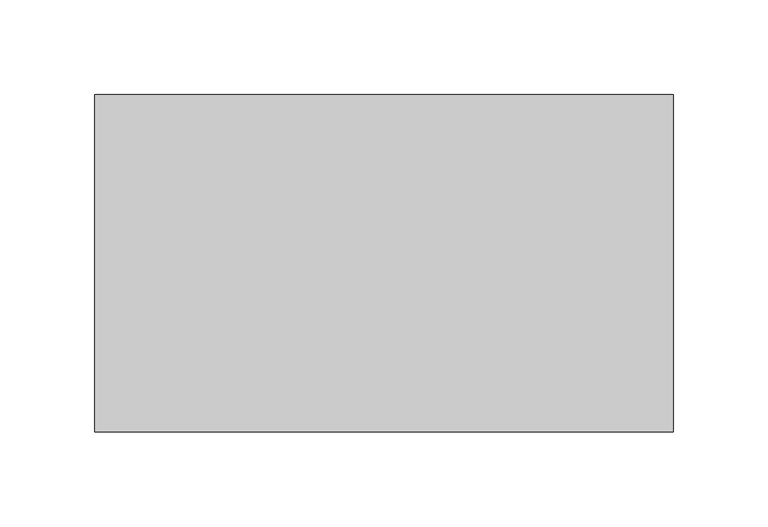
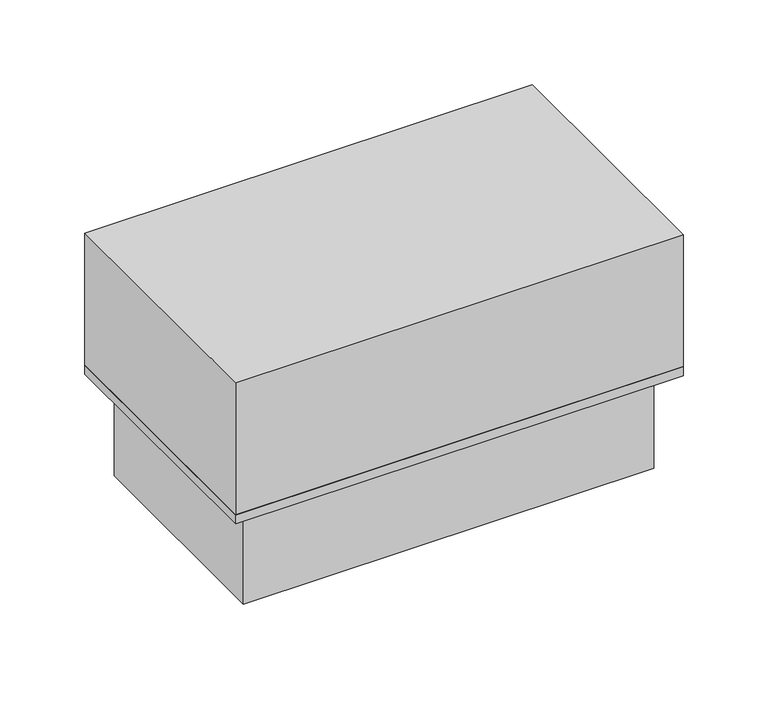
"""IFC4 building model written with IfcOpenShell, lengths in millimetres: proxy geometry, A4015 - Clock, Elapsed Time, Electric : A4015 - Clock, Elapsed Time, Electric."""

import ifcopenshell
import ifcopenshell.guid

model = None  # the IFC model being written
_history = None  # IfcOwnerHistory: only IFC2X3 demands one
_inside = {}  # id of a spatial element -> (the spatial element, [elements in it])
_under = {}  # id of a project, library or spatial element -> (it, [spatial elements below it])
_declared = {}  # id of a project -> (the project, [libraries it declares])
_typed = {}  # id of a type object -> (the type object, [elements of that type])
_made_of = {}  # id of a material, layer set ... -> (it, [elements and type objects made of it])


def new_model(schema):
    """Start an empty IFC model of exactly this schema.

    Asked for "IFC4X3", IfcOpenShell would pick the latest addendum, in which some entities
    have other attributes; the version numbers below select the first issue.
    IFC2X3 requires an IfcOwnerHistory on every rooted entity: one is made here for all.
    """
    global model, _history
    if schema == "IFC4X3":
        model = ifcopenshell.file(schema_version=(4, 3, 0, 0))
    else:
        model = ifcopenshell.file(schema=schema)
    _inside.clear()
    _under.clear()
    _declared.clear()
    _typed.clear()
    _made_of.clear()
    _history = None
    if model.schema == "IFC2X3":
        org = make("IfcOrganization", Name="unknown")
        user = make(
            "IfcPersonAndOrganization",
            ThePerson=make("IfcPerson", FamilyName="unknown"),
            TheOrganization=org,
        )
        app = make(
            "IfcApplication",
            ApplicationDeveloper=org,
            Version="unknown",
            ApplicationFullName="unknown",
            ApplicationIdentifier="unknown",
        )
        _history = make(
            "IfcOwnerHistory",
            OwningUser=user,
            OwningApplication=app,
            ChangeAction="ADDED",
            CreationDate=0,
        )
    return model


def make(cls, **values):
    """One entity of the class cls with the attributes given. An attribute that is None is left unset."""
    return model.create_entity(
        cls, **{name: value for name, value in values.items() if value is not None}
    )


def rooted(cls, **values):
    """An entity with a GlobalId (a new one), such as an element, a storey or a relation."""
    return make(cls, GlobalId=ifcopenshell.guid.new(), OwnerHistory=_history, **values)


def si_unit(unit_type, name, prefix=None):
    """IfcSIUnit, for example si_unit("LENGTHUNIT", "METRE", prefix="MILLI")."""
    return make("IfcSIUnit", UnitType=unit_type, Prefix=prefix, Name=name)


def assignment(units):
    """IfcUnitAssignment: the units of a project."""
    return None if units is None else make("IfcUnitAssignment", Units=units)


def point(xyz):
    """IfcCartesianPoint."""
    return None if xyz is None else make("IfcCartesianPoint", Coordinates=xyz)


def direction(xyz):
    """IfcDirection."""
    return None if xyz is None else make("IfcDirection", DirectionRatios=xyz)


def frame(location, z_axis=None, x_axis=None):
    """IfcAxis2Placement3D, a coordinate frame: its origin and axes. An axis left out is left unset."""
    return make(
        "IfcAxis2Placement3D",
        Location=point(location),
        Axis=direction(z_axis),
        RefDirection=direction(x_axis),
    )


def origin():
    """The frame at (0, 0, 0) with its axes left unset."""
    return frame((0.0, 0.0, 0.0))


def origin_with_axes():
    """The frame at (0, 0, 0) with the z axis (0, 0, 1) and the x axis (1, 0, 0) written out."""
    return frame((0.0, 0.0, 0.0), z_axis=(0.0, 0.0, 1.0), x_axis=(1.0, 0.0, 0.0))


def place(relative_to, where):
    """IfcLocalPlacement: puts the frame where relative to a parent placement (None: the world)."""
    return make(
        "IfcLocalPlacement", PlacementRelTo=relative_to, RelativePlacement=where
    )


def context(
    kind, dimensions, precision=None, world=None, true_north=None, identifier=None
):
    """IfcGeometricRepresentationContext, for example the 3D "Model" context."""
    return make(
        "IfcGeometricRepresentationContext",
        ContextIdentifier=identifier,
        ContextType=kind,
        CoordinateSpaceDimension=dimensions,
        Precision=precision,
        WorldCoordinateSystem=world,
        TrueNorth=true_north,
    )


def project(units=None, contexts=None):
    """IfcProject with its units and contexts."""
    return rooted(
        "IfcProject",
        Name="project",
        RepresentationContexts=contexts,
        UnitsInContext=assignment(units),
    )


def spatial(cls, under=None, at=None, **own):
    """A site, building, storey or space (cls), placed at a placement, below another one or the project."""
    s = rooted(cls, ObjectPlacement=at, **own)
    if under is not None:
        _under.setdefault(under.id(), (under, []))[1].append(s)
    return s


def polyline(points):
    """IfcPolyline through the points."""
    return make("IfcPolyline", Points=[point(p) for p in points])


def outline(outer, holes=None, kind="AREA"):
    """IfcArbitraryClosedProfileDef: a profile drawn as a closed curve; with holes, ...WithVoids."""
    if holes is None:
        return make("IfcArbitraryClosedProfileDef", ProfileType=kind, OuterCurve=outer)
    return make(
        "IfcArbitraryProfileDefWithVoids",
        ProfileType=kind,
        OuterCurve=outer,
        InnerCurves=holes,
    )


def extrude(swept, where, along, depth):
    """IfcExtrudedAreaSolid: the profile swept, set in the frame where, extruded along a direction by depth."""
    return make(
        "IfcExtrudedAreaSolid",
        SweptArea=swept,
        Position=where,
        ExtrudedDirection=direction(along),
        Depth=depth,
    )


def shape(context_of_items, identifier, shape_type, items):
    """IfcShapeRepresentation: the items that make up one representation, for example the "Body"."""
    return make(
        "IfcShapeRepresentation",
        ContextOfItems=context_of_items,
        RepresentationIdentifier=identifier,
        RepresentationType=shape_type,
        Items=items,
    )


def source(mapping_origin, context_of_items, identifier, shape_type, items):
    """IfcRepresentationMap: a shape defined once, which mapped items show again and again."""
    return make(
        "IfcRepresentationMap",
        MappingOrigin=mapping_origin,
        MappedRepresentation=shape(context_of_items, identifier, shape_type, items),
    )


def transform(
    local_origin,
    x_axis=None,
    y_axis=None,
    z_axis=None,
    scale=None,
    scale2=None,
    scale3=None,
    uniform=True,
):
    """IfcCartesianTransformationOperator3D, or its non-uniform kind. x_axis, y_axis, z_axis: its Axis1, 2, 3."""
    if uniform:
        return make(
            "IfcCartesianTransformationOperator3D",
            Axis1=direction(x_axis),
            Axis2=direction(y_axis),
            LocalOrigin=point(local_origin),
            Scale=scale,
            Axis3=direction(z_axis),
        )
    return make(
        "IfcCartesianTransformationOperator3DnonUniform",
        Axis1=direction(x_axis),
        Axis2=direction(y_axis),
        LocalOrigin=point(local_origin),
        Scale=scale,
        Axis3=direction(z_axis),
        Scale2=scale2,
        Scale3=scale3,
    )


def mapped(mapping_source, mapping_target):
    """IfcMappedItem: shows the shape of a source again, moved by a transform."""
    return make(
        "IfcMappedItem", MappingSource=mapping_source, MappingTarget=mapping_target
    )


def made_of(thing, what):
    """Note that an element or type object is made of a material, layer set ...; save() writes the relation."""
    if what is not None:
        _made_of.setdefault(what.id(), (what, []))[1].append(thing)
    return thing


def element(
    cls,
    number,
    at=None,
    inside=None,
    cuts=None,
    type_object=None,
    material=None,
    context=None,
    identifier="Body",
    shape_type=None,
    held_by="IfcProductDefinitionShape",
    body=None,
    shapes=None,
    **own,
):
    """One element of the class cls, such as IfcWall. Its Tag is "e" and its number.

    at: its placement. inside: the storey or other place that contains it. cuts: it is an
    opening in that element (IfcRelVoidsElement). A single representation is given by context,
    identifier, shape_type and body (its items); several are given by shapes. held_by: the class
    of the entity that holds the representations. save() writes the other relations.
    """
    e = rooted(cls, Tag="e%d" % number, ObjectPlacement=at, **own)
    if body is not None:
        shapes = [shape(context, identifier, shape_type, body)]
    if shapes is not None:
        e.Representation = make(held_by, Representations=shapes)
    if inside is not None:
        _inside.setdefault(inside.id(), (inside, []))[1].append(e)
    if cuts is not None:
        rooted(
            "IfcRelVoidsElement", RelatingBuildingElement=cuts, RelatedOpeningElement=e
        )
    if type_object is not None:
        _typed.setdefault(type_object.id(), (type_object, []))[1].append(e)
    return made_of(e, material)


def aggregate(whole, parts):
    """IfcRelAggregates: a whole, such as a stair, and the parts it consists of."""
    return rooted("IfcRelAggregates", RelatingObject=whole, RelatedObjects=parts)


def save(model, path):
    """Write the relations noted so far, then the file.

    IfcRelAggregates (storeys below a building ...), IfcRelContainedInSpatialStructure (elements
    in a storey), IfcRelDefinesByType, IfcRelAssociatesMaterial and IfcRelDeclares: one each for
    every whole, place, type object, material and project.
    """
    for whole, parts in _under.values():
        aggregate(whole, parts)
    for where, things in _inside.values():
        rooted(
            "IfcRelContainedInSpatialStructure",
            RelatedElements=things,
            RelatingStructure=where,
        )
    for kind, things in _typed.values():
        rooted("IfcRelDefinesByType", RelatedObjects=things, RelatingType=kind)
    for what, things in _made_of.values():
        rooted("IfcRelAssociatesMaterial", RelatedObjects=things, RelatingMaterial=what)
    for by, libraries in _declared.values():
        rooted("IfcRelDeclares", RelatingContext=by, RelatedDefinitions=libraries)
    model.write(path)


def specialty_equipment_8d654257(model_context):
    return source(origin(), model_context, "Body", "SweptSolid", [
        extrude(outline(polyline([(152.4, 0.0), (-152.4, 0.0), (-152.4, 177.8), (152.4, 177.8), (152.4, 0.0)])), origin_with_axes(), (0.0, 0.0, 1.0), 6.35),
        extrude(outline(polyline([(139.7, 12.7), (-139.7, 12.7), (-139.7, 165.1), (139.7, 165.1), (139.7, 12.7)])), frame((0.0, 0.0, -69.85), z_axis=(0.0, 0.0, 1.0), x_axis=(1.0, 0.0, 0.0)), (0.0, 0.0, 1.0), 69.85),
        extrude(outline(polyline([(152.4, 177.8), (152.4, 0.0), (-152.4, 0.0), (-152.4, 177.8), (152.4, 177.8)])), origin_with_axes(), (0.0, 0.0, 1.0), 101.6),
    ])


if __name__ == "__main__":
    model = new_model("IFC4")
    model_context = context("Model", 3, world=origin())
    ifc_project = project(units=[si_unit("LENGTHUNIT", "METRE", prefix="MILLI")], contexts=[model_context])
    site = spatial("IfcSite", under=ifc_project)
    building = spatial("IfcBuilding", under=site)
    placement = place(None, origin())
    specialty_equipment_shape = specialty_equipment_8d654257(model_context)
    element("IfcBuildingElementProxy", 1, Name="A4015 - Clock, Elapsed Time, Electric : A4015 - Clock, Elapsed Time, Electric", ObjectType="A4015 - Clock, Elapsed Time, Electric : A4015 - Clock, Elapsed Time, Electric", at=placement, inside=building, context=model_context, shape_type="MappedRepresentation", body=[
        mapped(specialty_equipment_shape, transform((0.0, 0.0, 0.0), x_axis=(1.0, 0.0, 0.0), y_axis=(0.0, 1.0, 0.0), z_axis=(0.0, 0.0, 1.0))),
    ])
    save(model, "model.ifc")

# Revit data of these elements
# Type "A4015 - Clock, Elapsed Time, Electric : A4015 - Clock, Elapsed Time, Electric"
#   Watts2 = "0"
#   Watts1 = "120"
#   Unit_Issue = "EA"
#   UTIL_6_Misc = "D"
#   UTIL_5_NonMedGas = "-"
#   UTIL_4_MiscGas = "-"
#   UTIL_3_MedGas = "-"
#   UTIL_2_Elec = "A"
#   UTIL_1_WaterDrain = "-"
#   Nomenclature = "Clock, Elapsed Time, Electric"
#   NSN = "6645"
#   Location [instance default] = ""
#   JSN = "A4015"
#   Fund_Source_VA = "-"
#   Fund_Source_Navy = "-"
#   Fund_Source_Army = "-"
#   Fund_Source_AF = "-"
#   ELEC_Volts2 = "0"
#   ELEC_Volts1 = "120"
#   ELEC_Phase2 = "0"
#   ELEC_Phase1 = "1"
#   ELEC_HertzSwitch = "0"
#   ELEC_HertzDependent = "-1"
#   ELEC_Hertz = "60"
#   ELEC_Amps2 = "0"
#   ELEC_Amps1 = "1"
#   DetailDescription = "Elapsed time digital electric clock. Single display time that can be used either as a clock or elapsed time indicator. Clock consists of buttons to set minutes, and hours for the time. For use in operating and delivery room, and medical service columns. Analog or digital displays may be provided as specified by the user."
#   CAT_VA = "A"
#   CAT_Navy = "A"
#   CAT_IHS = "-"
#   CAT_Army = "A"
#   CAT_AF = "A"
#   BTUperhour = "0"
#   Weight_IP = 3
#   Default Elevation = 6' - 6"
#   DIM_Width_IP = 1' - 0"
#   DIM_Height_IP = 0' - 7"
#   DIM_Depth_IP = 0' - 4"
# Element 1 (IfcBuildingElementProxy, "A4015 - Clock, Elapsed Time, Electric : A4015 - Clock, Elapsed Time, Electric")
#   Location = "LDDR1"
#   Materials on its faces: "EquipSpace"
# Materials
#   "EquipSpace": class "Unassigned", colour RGB 221 217 195, transparency 0.5
